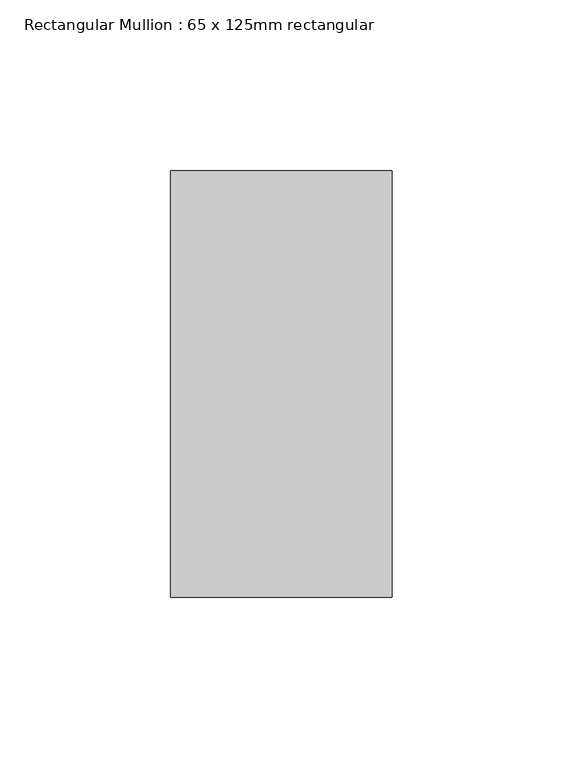
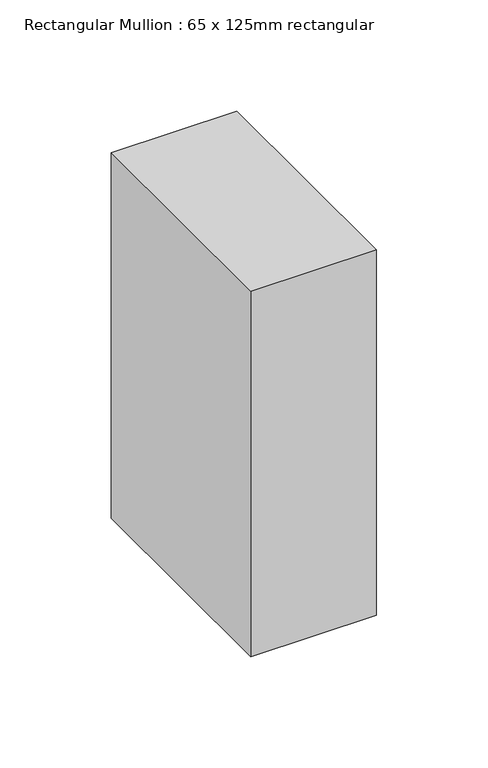
"""IFC4 building model written with IfcOpenShell, lengths in millimetres: member geometry, Rectangular Mullion : 65 x 125mm rectangular."""

import ifcopenshell
import ifcopenshell.guid

model = None  # the IFC model being written
_history = None  # IfcOwnerHistory: only IFC2X3 demands one
_inside = {}  # id of a spatial element -> (the spatial element, [elements in it])
_under = {}  # id of a project, library or spatial element -> (it, [spatial elements below it])
_declared = {}  # id of a project -> (the project, [libraries it declares])
_typed = {}  # id of a type object -> (the type object, [elements of that type])
_made_of = {}  # id of a material, layer set ... -> (it, [elements and type objects made of it])


def new_model(schema):
    """Start an empty IFC model of exactly this schema.

    Asked for "IFC4X3", IfcOpenShell would pick the latest addendum, in which some entities
    have other attributes; the version numbers below select the first issue.
    IFC2X3 requires an IfcOwnerHistory on every rooted entity: one is made here for all.
    """
    global model, _history
    if schema == "IFC4X3":
        model = ifcopenshell.file(schema_version=(4, 3, 0, 0))
    else:
        model = ifcopenshell.file(schema=schema)
    _inside.clear()
    _under.clear()
    _declared.clear()
    _typed.clear()
    _made_of.clear()
    _history = None
    if model.schema == "IFC2X3":
        org = make("IfcOrganization", Name="unknown")
        user = make(
            "IfcPersonAndOrganization",
            ThePerson=make("IfcPerson", FamilyName="unknown"),
            TheOrganization=org,
        )
        app = make(
            "IfcApplication",
            ApplicationDeveloper=org,
            Version="unknown",
            ApplicationFullName="unknown",
            ApplicationIdentifier="unknown",
        )
        _history = make(
            "IfcOwnerHistory",
            OwningUser=user,
            OwningApplication=app,
            ChangeAction="ADDED",
            CreationDate=0,
        )
    return model


def make(cls, **values):
    """One entity of the class cls with the attributes given. An attribute that is None is left unset."""
    return model.create_entity(
        cls, **{name: value for name, value in values.items() if value is not None}
    )


def rooted(cls, **values):
    """An entity with a GlobalId (a new one), such as an element, a storey or a relation."""
    return make(cls, GlobalId=ifcopenshell.guid.new(), OwnerHistory=_history, **values)


def si_unit(unit_type, name, prefix=None):
    """IfcSIUnit, for example si_unit("LENGTHUNIT", "METRE", prefix="MILLI")."""
    return make("IfcSIUnit", UnitType=unit_type, Prefix=prefix, Name=name)


def assignment(units):
    """IfcUnitAssignment: the units of a project."""
    return None if units is None else make("IfcUnitAssignment", Units=units)


def point(xyz):
    """IfcCartesianPoint."""
    return None if xyz is None else make("IfcCartesianPoint", Coordinates=xyz)


def direction(xyz):
    """IfcDirection."""
    return None if xyz is None else make("IfcDirection", DirectionRatios=xyz)


def frame(location, z_axis=None, x_axis=None):
    """IfcAxis2Placement3D, a coordinate frame: its origin and axes. An axis left out is left unset."""
    return make(
        "IfcAxis2Placement3D",
        Location=point(location),
        Axis=direction(z_axis),
        RefDirection=direction(x_axis),
    )


def origin():
    """The frame at (0, 0, 0) with its axes left unset."""
    return frame((0.0, 0.0, 0.0))


def place(relative_to, where):
    """IfcLocalPlacement: puts the frame where relative to a parent placement (None: the world)."""
    return make(
        "IfcLocalPlacement", PlacementRelTo=relative_to, RelativePlacement=where
    )


def context(
    kind, dimensions, precision=None, world=None, true_north=None, identifier=None
):
    """IfcGeometricRepresentationContext, for example the 3D "Model" context."""
    return make(
        "IfcGeometricRepresentationContext",
        ContextIdentifier=identifier,
        ContextType=kind,
        CoordinateSpaceDimension=dimensions,
        Precision=precision,
        WorldCoordinateSystem=world,
        TrueNorth=true_north,
    )


def project(units=None, contexts=None):
    """IfcProject with its units and contexts."""
    return rooted(
        "IfcProject",
        Name="project",
        RepresentationContexts=contexts,
        UnitsInContext=assignment(units),
    )


def spatial(cls, under=None, at=None, **own):
    """A site, building, storey or space (cls), placed at a placement, below another one or the project."""
    s = rooted(cls, ObjectPlacement=at, **own)
    if under is not None:
        _under.setdefault(under.id(), (under, []))[1].append(s)
    return s


def polyline(points):
    """IfcPolyline through the points."""
    return make("IfcPolyline", Points=[point(p) for p in points])


def outline(outer, holes=None, kind="AREA"):
    """IfcArbitraryClosedProfileDef: a profile drawn as a closed curve; with holes, ...WithVoids."""
    if holes is None:
        return make("IfcArbitraryClosedProfileDef", ProfileType=kind, OuterCurve=outer)
    return make(
        "IfcArbitraryProfileDefWithVoids",
        ProfileType=kind,
        OuterCurve=outer,
        InnerCurves=holes,
    )


def extrude(swept, where, along, depth):
    """IfcExtrudedAreaSolid: the profile swept, set in the frame where, extruded along a direction by depth."""
    return make(
        "IfcExtrudedAreaSolid",
        SweptArea=swept,
        Position=where,
        ExtrudedDirection=direction(along),
        Depth=depth,
    )


def shape(context_of_items, identifier, shape_type, items):
    """IfcShapeRepresentation: the items that make up one representation, for example the "Body"."""
    return make(
        "IfcShapeRepresentation",
        ContextOfItems=context_of_items,
        RepresentationIdentifier=identifier,
        RepresentationType=shape_type,
        Items=items,
    )


def source(mapping_origin, context_of_items, identifier, shape_type, items):
    """IfcRepresentationMap: a shape defined once, which mapped items show again and again."""
    return make(
        "IfcRepresentationMap",
        MappingOrigin=mapping_origin,
        MappedRepresentation=shape(context_of_items, identifier, shape_type, items),
    )


def transform(
    local_origin,
    x_axis=None,
    y_axis=None,
    z_axis=None,
    scale=None,
    scale2=None,
    scale3=None,
    uniform=True,
):
    """IfcCartesianTransformationOperator3D, or its non-uniform kind. x_axis, y_axis, z_axis: its Axis1, 2, 3."""
    if uniform:
        return make(
            "IfcCartesianTransformationOperator3D",
            Axis1=direction(x_axis),
            Axis2=direction(y_axis),
            LocalOrigin=point(local_origin),
            Scale=scale,
            Axis3=direction(z_axis),
        )
    return make(
        "IfcCartesianTransformationOperator3DnonUniform",
        Axis1=direction(x_axis),
        Axis2=direction(y_axis),
        LocalOrigin=point(local_origin),
        Scale=scale,
        Axis3=direction(z_axis),
        Scale2=scale2,
        Scale3=scale3,
    )


def mapped(mapping_source, mapping_target):
    """IfcMappedItem: shows the shape of a source again, moved by a transform."""
    return make(
        "IfcMappedItem", MappingSource=mapping_source, MappingTarget=mapping_target
    )


def made_of(thing, what):
    """Note that an element or type object is made of a material, layer set ...; save() writes the relation."""
    if what is not None:
        _made_of.setdefault(what.id(), (what, []))[1].append(thing)
    return thing


def element(
    cls,
    number,
    at=None,
    inside=None,
    cuts=None,
    type_object=None,
    material=None,
    context=None,
    identifier="Body",
    shape_type=None,
    held_by="IfcProductDefinitionShape",
    body=None,
    shapes=None,
    **own,
):
    """One element of the class cls, such as IfcWall. Its Tag is "e" and its number.

    at: its placement. inside: the storey or other place that contains it. cuts: it is an
    opening in that element (IfcRelVoidsElement). A single representation is given by context,
    identifier, shape_type and body (its items); several are given by shapes. held_by: the class
    of the entity that holds the representations. save() writes the other relations.
    """
    e = rooted(cls, Tag="e%d" % number, ObjectPlacement=at, **own)
    if body is not None:
        shapes = [shape(context, identifier, shape_type, body)]
    if shapes is not None:
        e.Representation = make(held_by, Representations=shapes)
    if inside is not None:
        _inside.setdefault(inside.id(), (inside, []))[1].append(e)
    if cuts is not None:
        rooted(
            "IfcRelVoidsElement", RelatingBuildingElement=cuts, RelatedOpeningElement=e
        )
    if type_object is not None:
        _typed.setdefault(type_object.id(), (type_object, []))[1].append(e)
    return made_of(e, material)


def aggregate(whole, parts):
    """IfcRelAggregates: a whole, such as a stair, and the parts it consists of."""
    return rooted("IfcRelAggregates", RelatingObject=whole, RelatedObjects=parts)


def save(model, path):
    """Write the relations noted so far, then the file.

    IfcRelAggregates (storeys below a building ...), IfcRelContainedInSpatialStructure (elements
    in a storey), IfcRelDefinesByType, IfcRelAssociatesMaterial and IfcRelDeclares: one each for
    every whole, place, type object, material and project.
    """
    for whole, parts in _under.values():
        aggregate(whole, parts)
    for where, things in _inside.values():
        rooted(
            "IfcRelContainedInSpatialStructure",
            RelatedElements=things,
            RelatingStructure=where,
        )
    for kind, things in _typed.values():
        rooted("IfcRelDefinesByType", RelatedObjects=things, RelatingType=kind)
    for what, things in _made_of.values():
        rooted("IfcRelAssociatesMaterial", RelatedObjects=things, RelatingMaterial=what)
    for by, libraries in _declared.values():
        rooted("IfcRelDeclares", RelatingContext=by, RelatedDefinitions=libraries)
    model.write(path)


def rectangular_mullion_65_x_125mm_rectangular_470365d3(model_context):
    return source(origin(), model_context, "Body", "SweptSolid", [
        extrude(outline(polyline([(32.5, 62.5), (32.5, -62.5), (-32.5, -62.5), (-32.5, 62.5), (32.5, 62.5)])), frame((0.0, 0.0, -200.0), z_axis=(0.0, 0.0, 1.0), x_axis=(1.0, 0.0, 0.0)), (0.0, 0.0, 1.0), 200.0),
    ])


if __name__ == "__main__":
    model = new_model("IFC4")
    model_context = context("Model", 3, world=origin())
    ifc_project = project(units=[si_unit("LENGTHUNIT", "METRE", prefix="MILLI")], contexts=[model_context])
    site = spatial("IfcSite", under=ifc_project)
    building = spatial("IfcBuilding", under=site)
    placement = place(None, origin())
    rectangular_mullion_65_x_125mm_rectangular_shape = rectangular_mullion_65_x_125mm_rectangular_470365d3(model_context)
    element("IfcMember", 1, ObjectType="Rectangular Mullion : 65 x 125mm rectangular", at=placement, inside=building, context=model_context, shape_type="MappedRepresentation", body=[
        mapped(rectangular_mullion_65_x_125mm_rectangular_shape, transform((0.0, 0.0, 0.0), x_axis=(1.0, 0.0, 0.0), y_axis=(0.0, 1.0, 0.0), z_axis=(0.0, 0.0, 1.0))),
    ])
    save(model, "model.ifc")

# Revit data of these elements
# Type "Rectangular Mullion : 65 x 125mm rectangular"
#   built-in parameter 1007304 = 0.410105 (stored number, unit not read)
#   built-in parameter 1007301 = 0.106627 (stored number, unit not read)
#   built-in parameter 1007300 = 0.106627 (stored number, unit not read)
# Element 1 (IfcMember, "Rectangular Mullion : 65 x 125mm rectangular")
#   Materials on its faces: "Aluminum"
# Materials
#   "Aluminum": class "Metal", colour RGB 244 245 246, transparency 0, Description = "Aluminum 6061", Cost = 0
